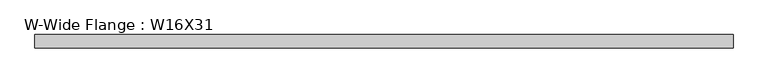
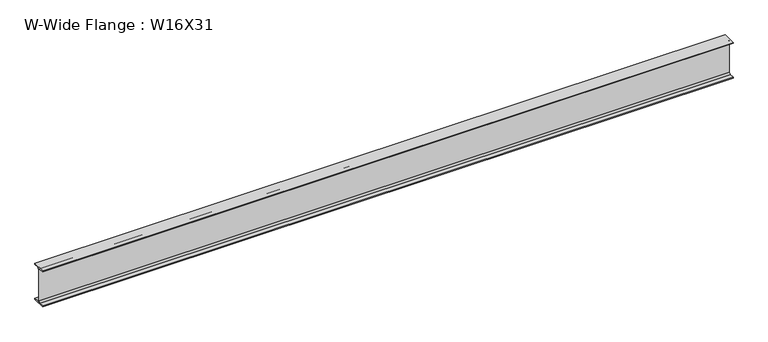
"""IFC4 building model written with IfcOpenShell, lengths in millimetres: beam geometry, W-Wide Flange : W16X31."""

from ifc_helpers import new_model, si_unit, point, frame, frame_2d, origin, place, context, project, spatial, polyline, circle_curve, trimmed, segment, composite_curve, outline, extrude, source, transform, mapped, element, save


def w_wide_flange_w16x31_013d4ff7(model_context):
    return source(origin(), model_context, "Body", "SweptSolid", [
        extrude(outline(composite_curve([segment(polyline([(70.231, -190.754), (70.231, -201.93), (-70.231, -201.93), (-70.231, -190.754), (-20.8915, -190.754)]), True, "CONTINUOUS"), segment(trimmed(circle_curve(frame_2d((-20.8915, -173.355)), 17.399), [point((-20.8915, -190.754))], [point((-3.4925, -173.355))], True, "CARTESIAN"), True, "CONTINUOUS"), segment(polyline([(-3.4925, -173.355), (-3.4925, 173.355)]), True, "CONTINUOUS"), segment(trimmed(circle_curve(frame_2d((-20.8915, 173.355)), 17.399), [point((-3.4925, 173.355))], [point((-20.8915, 190.754))], True, "CARTESIAN"), True, "CONTINUOUS"), segment(polyline([(-20.8915, 190.754), (-70.231, 190.754), (-70.231, 201.93), (70.231, 201.93), (70.231, 190.754), (20.8915, 190.754)]), True, "CONTINUOUS"), segment(trimmed(circle_curve(frame_2d((20.8915, 173.355)), 17.399), [point((20.8915, 190.754))], [point((3.4925, 173.355))], True, "CARTESIAN"), True, "CONTINUOUS"), segment(polyline([(3.4925, 173.355), (3.4925, -173.355)]), True, "CONTINUOUS"), segment(trimmed(circle_curve(frame_2d((20.8915, -173.355)), 17.399), [point((3.4925, -173.355))], [point((20.8915, -190.754))], True, "CARTESIAN"), True, "CONTINUOUS"), segment(polyline([(20.8915, -190.754), (70.231, -190.754)]), True, "CONTINUOUS")], self_intersect=False)), frame((-3613.7120876, 0.0, 0.0), z_axis=(1.0, 0.0, 0.0), x_axis=(0.0, 1.0, 0.0)), (0.0, 0.0, 1.0), 7328.9404921),
    ])


if __name__ == "__main__":
    model = new_model("IFC4")
    model_context = context("Model", 3, world=origin())
    ifc_project = project(units=[si_unit("LENGTHUNIT", "METRE", prefix="MILLI")], contexts=[model_context])
    site = spatial("IfcSite", under=ifc_project)
    building = spatial("IfcBuilding", under=site)
    placement = place(None, origin())
    w_wide_flange_w16x31_shape = w_wide_flange_w16x31_013d4ff7(model_context)
    element("IfcBeam", 1, ObjectType="W-Wide Flange : W16X31", at=placement, inside=building, context=model_context, shape_type="MappedRepresentation", body=[
        mapped(w_wide_flange_w16x31_shape, transform((0.0, 0.0, 0.0), x_axis=(1.0, 0.0, 0.0), y_axis=(0.0, 1.0, 0.0), z_axis=(0.0, 0.0, 1.0))),
    ])
    save(model, "model.ifc")

# Revit data of these elements
# Type "W-Wide Flange : W16X31"
#   Assembly Code = "B10"
#   W = 31
#   Start Extension Calculation [instance default] = 10' - 0"
#   Start Extension [instance default] = -0' - 0 1/2"
#   End Extension Calculation [instance default] = 10' - 0"
#   End Extension [instance default] = -0' - 0 1/2"
#   Length [instance default] = 5' - 0"
#   bf = 0' - 5.53"
#   d = 1' - 3.9"
#   k = 0' - 1 1/8"
#   k2 = 0' - 0.685"
#   tf = 0' - 0.44"
#   tw = 0' - 0.275"
#   A = 0.0634028 SF
#   Beam Material [instance default] = Metal - Steel - ASTM A992
# Element 1 (IfcBeam, "W-Wide Flange : W16X31")
#   Materials on its faces: "Metal - Steel - ASTM A992"
# Materials
#   "Metal - Steel - ASTM A992": class "Metal", colour RGB 128 0 0, transparency 0
